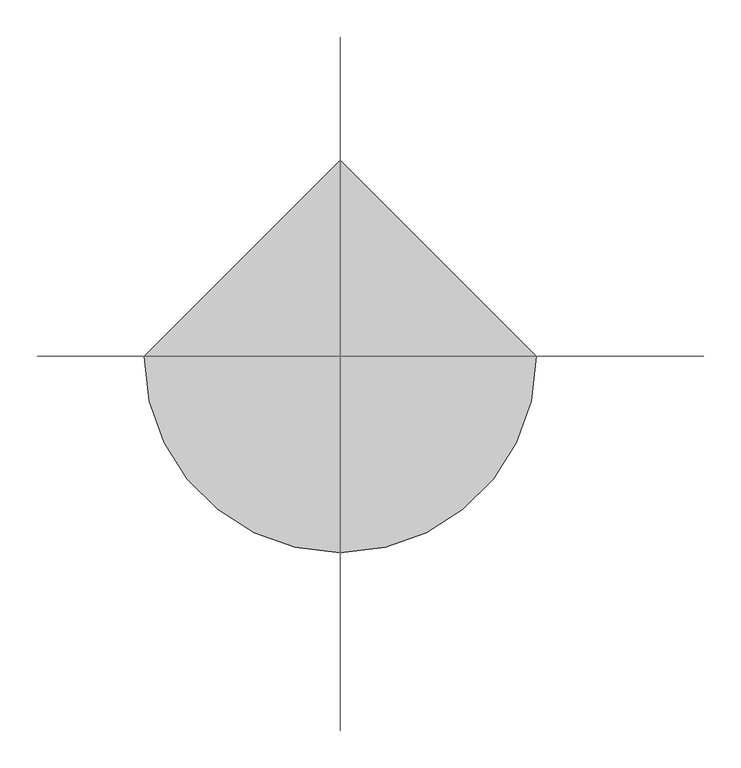
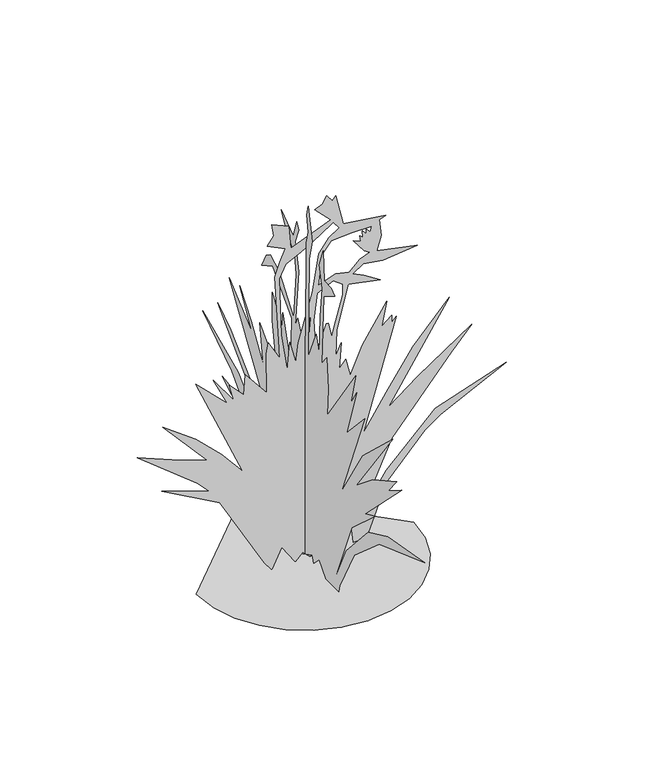
"""IFC4 building model written with IfcOpenShell, lengths in millimetres: proxy geometry, crane lily 26101 : crane lily 26101."""

from ifc_helpers import new_model, si_unit, origin, place, context, project, spatial, triangles, source, transform, mapped, element, save


def entourage_55f6ff97(model_context):
    return source(origin(), model_context, "Body", "Tessellation", [
        triangles([(-264.3380075, 0.0, 0.0272524), (-257.3504617, -60.5688865, 0.0272524), (-237.4475159, -116.1916269, 0.0272524), (-206.2245489, -165.274632, 0.0272524), (-165.274632, -206.2245489, 0.0272524), (-116.1916269, -237.4475159, 0.0272524), (-60.5688865, -257.3504617, 0.0272524), (1.16e-05, -264.3380075, 0.0272524), (60.5688865, -257.3504617, 0.0272524), (116.1916269, -237.4475159, 0.0272524), (165.274632, -206.2245489, 0.0272524), (206.2245489, -165.274632, 0.0272524), (237.4475159, -116.1916269, 0.0272524), (257.3504617, -60.5688865, 0.0272524), (264.3380075, 2.31e-05, 0.0272524), (-3.47e-05, 264.3380075, 0.0272524), (-5.2e-06, -141.3706678, 0.0), (-2.8e-06, -89.4159448, 0.054498), (-3.14e-05, -59.9343958, 33.2735186), (-3.1e-05, -36.3827356, 9.846953), (-3.03e-05, -30.3380374, 26.1345898), (2.2e-06, 22.1351019, 0.0353721), (-2.75e-05, 35.0893666, 22.475361), (-2.7e-05, 50.4325003, 13.9824575), (-2.41e-05, 71.8028075, 80.7852761), (5.2e-06, 91.613049, 0.0211753), (-2.36e-05, 109.0153662, 40.8424698), (-2.42e-05, 112.8357816, 15.9965016), (-1.83e-05, 164.4437961, 134.5614359), (-1.5e-05, 201.3025201, 190.8125718), (-8.6e-06, 314.8967674, 236.0083596), (-6.4e-06, 348.2342674, 257.8737037), (-8.8e-06, 301.5160253, 250.5209003), (-1.18e-05, 246.732487, 231.9590791), (-7.1e-06, 309.0598417, 295.0364789), (8e-07, 430.3017509, 376.6543714), (-7.9e-06, 280.4721063, 309.3519387), (-1.58e-05, 174.5674878, 204.3200503), (-9.8e-06, 240.1660818, 307.4037292), (-3e-07, 367.670363, 434.9626582), (-3.8e-06, 312.5929836, 399.2629114), (-1.14e-05, 210.1351387, 300.3374635), (-1.65e-05, 148.1844779, 220.8381918), (-1.17e-05, 187.1702069, 323.3016323), (3e-07, 320.1596366, 527.8276657), (-6.4e-06, 222.976615, 445.7627257), (-1.5e-06, 274.807899, 534.3072121), (-5.5e-06, 226.7299833, 472.9153562), (-1.02e-05, 175.4651256, 391.7724529), (-6.5e-06, 190.5821898, 491.1144633), (-1.2e-05, 119.3145649, 415.5265626), (-7.8e-06, 137.4532288, 529.6031387), (-5.6e-06, 138.7511692, 601.2540341), (-9.5e-06, 94.9513718, 536.1969586), (-8.4e-06, 93.3989229, 575.3383922), (-1.32e-05, 59.5732078, 463.4487828), (-9.8e-06, 56.2066891, 583.9388483), (-3.7e-06, 136.0049161, 669.1432405), (-2.4e-06, 181.9436545, 644.4467829), (-2.1e-06, 163.9243692, 680.6875214), (-2.5e-06, 147.0399529, 691.5511024), (-4.8e-06, 108.1804607, 671.9067347), (-1e-05, 48.046931, 590.4565101), (-6.9e-06, 36.8709235, 709.0745968), (-5.3e-06, 43.8627887, 753.7100264), (-2e-06, 83.7514831, 804.4440662), (-3e-07, 99.8779606, 836.6538008), (-3.7e-06, 49.136086, 799.8898384), (-2.9e-06, 35.0893666, 845.2923723), (-3.8e-06, 26.4505657, 828.0152292), (-4.3e-06, 41.5678933, 791.3020632), (-7e-06, 26.8495989, 721.233593), (-1.07e-05, 41.5678933, 575.3383922), (-1.05e-05, 30.7698379, 599.0950453), (-1.29e-05, 9.1735731, 551.5843188), (-1.27e-05, -4.2437592, 577.167205), (-5.7e-06, -6.2811965, 815.731822), (-5.1e-06, -13.569935, 847.4513248), (-3.6e-06, -6.9461944, 887.7586756), (-3.1e-06, -14.582304, 914.4007267), (-6.2e-06, -30.3001922, 833.2324253), (-7.2e-06, -17.1413308, 780.7407166), (-1.46e-05, -14.582304, 527.8276657), (-1.38e-05, -46.9765748, 605.5745916), (-1.57e-05, -59.9343958, 560.222854), (-1.28e-05, -63.7807226, 662.0591526), (-1.1e-05, -73.6229771, 738.5157503), (-8.8e-06, -59.9343958, 791.3020632), (-8.5e-06, -68.5729447, 815.05868), (-8.2e-06, -77.2114935, 838.812826), (-1.06e-05, -81.5307611, 763.227396), (-1.2e-05, -110.9300204, 761.8202871), (-1.3e-05, -126.4778813, 751.5510738), (-1.23e-05, -100.3333834, 735.2899298), (-1.17e-05, -79.708316, 722.0590513), (-1.66e-05, -70.7324513, 545.1047725), (-1.68e-05, -92.3897821, 572.3361045), (-1.94e-05, -98.8076044, 495.4324774), (-2.12e-05, -94.4883277, 426.3240867), (-2.14e-05, -213.2677237, 599.0950453), (-2.3e-05, -193.8311193, 517.0301053), (-2.28e-05, -217.5869913, 558.0613217), (-2.48e-05, -176.5542669, 430.6446442), (-2.57e-05, -252.1411685, 512.7095841), (-2.87e-05, -152.798395, 264.3532501), (-2.83e-05, -244.4081376, 413.0424482), (-3.04e-05, -369.3264393, 531.0712541), (-2.98e-05, -215.4274755, 318.343541), (-3.13e-05, -285.475907, 376.1107999), (-3.42e-05, -387.58906, 431.8587779), (-3.39e-05, -351.4829427, 387.4518954), (-3.53e-05, -406.9616784, 422.1127885), (-3.3e-05, -254.1018046, 269.3443517), (-3.43e-05, -295.3336628, 288.109885), (-3.26e-05, -197.6014924, 198.8161167), (-3.48e-05, -118.2442087, 7.3579794), (-3.37e-05, -173.2017281, 125.4509545), (-3.48e-05, -266.8272088, 229.6761334), (-3.73e-05, -347.9879162, 267.302198), (-4.35e-05, -504.8177693, 294.5894314), (-3.69e-05, -312.1281501, 226.3418711), (-3.5e-05, -207.3218293, 133.5593986), (-3.57e-05, -146.3193573, 18.1561127), (117.3305654, 2.31e-05, 0.0405123), (110.3389591, 2.08e-05, 74.4091073), (78.0842327, 2.54e-05, 21.0145808), (55.6151237, 2.49e-05, 46.2313396), (12.5873108, 2.89e-05, 0.0122306), (-5.1707583, 2.92e-05, 18.1490262), (-24.1045425, 3.09e-05, 0.0037426), (-56.6857342, 2.97e-05, 48.3908508), (-81.2114855, 3.28e-05, 0.0181663), (-98.986418, 3.3e-05, 24.1438615), (-207.7917316, 2.63e-05, 216.6390658), (-348.2342674, 2.78e-05, 294.5894314), (-233.774666, 2.51e-05, 255.7146967), (-261.6024369, 2.45e-05, 285.2828592), (-408.7041229, 2.4e-05, 402.5700133), (-324.6782925, 2.24e-05, 368.0386909), (-238.0939517, 2.05e-05, 335.6206115), (-346.0752786, 1.79e-05, 458.719275), (-266.2303157, 1.79e-05, 400.2179767), (-203.8244956, 1.88e-05, 339.715129), (-151.7089902, 2.02e-05, 277.3123428), (-266.1693456, 9.5e-06, 540.784215), (-189.3886398, 1.06e-05, 466.0141786), (-222.976615, 7.9e-06, 536.4662009), (-173.7341084, 9.8e-06, 467.1774796), (-184.1031521, 7.7e-06, 510.5505589), (-149.5492202, 8.4e-06, 473.8373929), (-145.2299525, 5.2e-06, 523.5096517), (-93.3989229, 6.8e-06, 458.719275), (-94.0984351, 9e-07, 559.4354384), (-89.0799006, -9e-07, 586.138496), (-61.0044976, 8e-07, 536.4662009), (-64.4230889, -1.9e-06, 583.7153154), (-73.364658, -1.14e-05, 749.2980864), (-61.7167134, -1.39e-05, 783.3111992), (-47.9079951, -1.63e-05, 813.4864649), (-91.2394163, -1.57e-05, 834.4947756), (-76.5455003, -1.76e-05, 856.3946743), (-80.4413563, -1.92e-05, 886.3260595), (-39.8899707, -2e-05, 869.0464457), (-35.0893666, -1.67e-05, 810.7381588), (62.093907, -2.33e-05, 849.6128935), (23.2207756, -2.39e-05, 888.4850847), (42.4165107, -2.52e-05, 896.5013105), (53.4556125, -2.67e-05, 914.4007267), (66.1944834, -2.63e-05, 896.8848627), (74.7598808, -2.72e-05, 906.7806976), (93.6785752, -2.34e-05, 828.1498867), (196.1872255, -2.7e-05, 813.9157265), (180.8732984, -2.6e-05, 808.5791336), (185.7325766, -2.37e-05, 766.8723043), (174.394515, -2.11e-05, 730.8322803), (273.7385602, -2.41e-05, 709.2371595), (189.3833167, -2e-05, 700.9592491), (142.0676456, -1.83e-05, 708.1576469), (116.0844387, -1.62e-05, 691.9600891), (142.8525086, -1.66e-05, 679.102589), (183.0330503, -1.68e-05, 653.0853544), (105.3178811, -1.44e-05, 669.0848139), (77.0491851, -6.7e-06, 560.5047772), (75.051728, -2.7e-06, 495.4324774), (87.9216592, -5e-06, 524.393573), (83.6900225, -9e-07, 458.719275), (98.8076044, -2.7e-06, 478.1553706), (109.6056554, -5e-07, 432.803633), (138.9439536, -5.8e-06, 499.7708027), (199.0078928, -1.39e-05, 592.0084502), (187.352336, -9.8e-06, 532.1482232), (211.1082079, -1.2e-05, 551.5843188), (211.1082079, -1.1e-05, 534.3072121), (221.9062589, -1.21e-05, 545.1047725), (142.0000807, 7.6e-06, 272.9918035), (197.3987977, 1e-07, 358.912431), (262.4025334, -8.4e-06, 452.8214155), (351.4829427, -1.8e-05, 549.4227502), (202.4694002, 2.3e-06, 318.343541), (273.8909673, -4.1e-06, 372.7275035), (405.4757589, -1.51e-05, 460.8783002), (355.6612487, -9.6e-06, 405.7856601), (211.5270596, 6.8e-06, 235.3906284), (131.6828507, 2.08e-05, 59.5396797), (197.4798247, 1.2e-05, 158.3333043), (317.0659301, -2e-07, 275.0161712), (489.6996878, -1.12e-05, 333.4616226), (330.1571005, 5e-07, 255.2422691), (291.8284444, 3.8e-06, 227.7759587), (199.2240496, 1.38e-05, 127.0808696), (148.478864, 2.13e-05, 0.0507429), (114.3788288, -2.24e-05, 797.4488537), (63.6714996, -2.01e-05, 794.7361559), (42.3199913, -1.75e-05, 767.5631779), (31.8592449, -1.25e-05, 691.9600891), (74.6966352, -1.53e-05, 706.3237473), (107.4461487, -1.62e-05, 698.437092), (132.807564, -1.88e-05, 722.7067589), (157.1176626, -2.05e-05, 732.9912329), (143.9299774, -2.04e-05, 741.276701), (117.5705943, -2.13e-05, 776.2906248), (135.9680906, -2.16e-05, 768.3049204), (133.7021497, -2.24e-05, 783.2401279), (140.693002, -2.24e-05, 777.0983517), (139.840574, -2.33e-05, 793.4610884), (148.478864, -2.3e-05, 782.6634916), (148.8047525, -2.38e-05, 795.162874), (158.4753014, -2.36e-05, 785.4854851), (162.2614257, -2.45e-05, 797.6698431), (36.4967821, -2.03e-05, 819.0008085), (-10.5179706, -1.66e-05, 790.7762959), (-46.6034508, -1.4e-05, 773.6338102), (-62.8378705, -1.14e-05, 741.9143074), (-57.6440741, -2.8e-06, 594.8100597), (-43.7276589, 2.2e-06, 499.7530349), (-37.2488755, -2.2e-06, 568.8613893), (-22.1313685, 5e-07, 512.7095841), (-15.8925131, -2.6e-06, 559.8647), (18.0916476, -1.1e-05, 677.0451565), (33.6138798, -1.74e-05, 772.2038103), (57.6697312, -2.04e-05, 805.3914648), (83.6900225, -2.25e-05, 821.5356829), (68.5729447, -2.3e-05, 840.9743219), (30.2087529, -1.13e-05, 671.65784), (21.8014718, -6.9e-06, 605.0462809), (25.6817059, -2.5e-06, 528.0867342), (30.8554363, -2.8e-06, 528.7344418), (51.5501011, -7.1e-06, 586.290885), (56.0771503, -7.3e-06, 585.6457209), (65.1309854, -5.4e-06, 548.1349654), (69.6580301, -6.8e-06, 568.1831966), (91.6460685, -1.24e-05, 645.7879074), (91.6460685, -1.4e-05, 672.9507116), (68.3644091, -1.4e-05, 690.4106197), (6.9271952, -5.7e-06, 595.3460009), (10.8074288, -4.5e-06, 573.3571904), (13.394269, -6.1e-06, 597.9317079), (15.3343985, -7.9e-06, 627.035055)], [[15, 16, 1], [14, 15, 1], [14, 1, 2], [13, 14, 2], [13, 2, 3], [13, 3, 4], [12, 13, 4], [11, 12, 4], [11, 4, 5], [11, 5, 6], [11, 6, 7], [11, 7, 8], [11, 8, 9], [11, 9, 10], [46, 47, 48], [119, 120, 121], [35, 36, 37], [106, 107, 108], [39, 40, 41], [39, 41, 42], [101, 102, 103], [111, 112, 113], [105, 106, 108], [44, 45, 46], [113, 114, 115], [54, 55, 56], [103, 104, 105], [99, 100, 101], [109, 110, 111], [89, 90, 91], [118, 119, 121], [31, 32, 33], [46, 48, 49], [44, 46, 49], [79, 80, 81], [78, 79, 81], [66, 67, 68], [27, 28, 29], [52, 53, 54], [88, 89, 91], [87, 88, 91], [49, 50, 51], [58, 59, 60], [99, 101, 103], [25, 26, 27], [83, 84, 85], [109, 111, 113], [108, 109, 113], [96, 97, 98], [68, 69, 70], [68, 70, 71], [38, 39, 42], [38, 42, 43], [65, 66, 68], [65, 68, 71], [65, 71, 72], [64, 65, 72], [64, 72, 73], [63, 64, 73], [118, 121, 122], [117, 118, 122], [117, 122, 123], [116, 117, 123], [73, 74, 75], [116, 123, 17], [116, 17, 18], [58, 60, 61], [58, 61, 62], [57, 58, 62], [57, 62, 63], [77, 78, 81], [77, 81, 82], [76, 77, 82], [76, 82, 83], [75, 76, 83], [92, 93, 94], [19, 20, 21], [30, 31, 33], [30, 33, 34], [91, 92, 94], [87, 91, 94], [87, 94, 95], [86, 87, 95], [86, 95, 96], [85, 86, 96], [34, 35, 37], [34, 37, 38], [30, 34, 38], [25, 27, 29], [57, 63, 73], [56, 57, 73], [56, 73, 75], [56, 75, 83], [23, 24, 25], [99, 103, 105], [29, 30, 38], [105, 108, 113], [105, 113, 115], [51, 52, 54], [51, 54, 56], [83, 85, 96], [21, 22, 23], [83, 96, 98], [83, 98, 99], [56, 83, 99], [29, 38, 43], [25, 29, 43], [115, 116, 18], [115, 18, 19], [105, 115, 19], [21, 23, 25], [44, 49, 51], [43, 44, 51], [56, 99, 105], [51, 56, 105], [43, 51, 105], [43, 105, 19], [25, 43, 19], [21, 25, 19], [248, 124, 125], [241, 229, 212], [206, 207, 208], [197, 198, 199], [146, 147, 148], [134, 135, 136], [196, 197, 199], [241, 212, 213], [255, 237, 238], [140, 141, 142], [200, 201, 202], [137, 138, 139], [255, 238, 239], [258, 255, 239], [175, 176, 177], [184, 185, 186], [235, 236, 237], [180, 181, 182], [189, 190, 191], [144, 145, 146], [140, 142, 143], [247, 248, 125], [171, 172, 173], [200, 202, 203], [199, 200, 203], [193, 194, 195], [237, 255, 256], [220, 221, 222], [148, 149, 150], [137, 139, 140], [224, 225, 226], [229, 241, 242], [195, 196, 199], [222, 223, 224], [153, 154, 155], [179, 180, 182], [150, 151, 152], [226, 227, 228], [191, 192, 193], [186, 187, 188], [169, 170, 171], [175, 177, 178], [152, 153, 155], [195, 199, 203], [161, 162, 163], [240, 241, 213], [240, 213, 214], [165, 166, 167], [167, 168, 169], [165, 167, 169], [165, 169, 171], [191, 193, 195], [189, 191, 195], [188, 189, 195], [239, 240, 214], [239, 214, 215], [125, 126, 127], [124, 248, 249], [124, 249, 250], [161, 163, 164], [160, 161, 164], [159, 160, 164], [131, 132, 133], [144, 146, 148], [129, 130, 131], [131, 133, 134], [206, 208, 209], [205, 206, 209], [205, 209, 210], [204, 205, 210], [204, 210, 211], [204, 211, 124], [204, 124, 250], [246, 247, 125], [195, 203, 204], [144, 148, 150], [144, 150, 152], [158, 159, 164], [127, 128, 129], [246, 125, 127], [246, 127, 129], [246, 129, 131], [136, 137, 140], [136, 140, 143], [136, 143, 144], [134, 136, 144], [131, 134, 144], [220, 222, 224], [220, 224, 226], [220, 226, 228], [219, 220, 228], [131, 144, 152], [258, 239, 215], [174, 175, 178], [186, 188, 195], [215, 216, 217], [131, 152, 155], [157, 158, 164], [217, 218, 219], [186, 195, 204], [219, 228, 229], [245, 246, 131], [245, 131, 215], [244, 245, 215], [254, 244, 215], [254, 215, 217], [253, 254, 217], [252, 253, 217], [257, 258, 215], [184, 186, 204], [184, 204, 250], [183, 184, 250], [183, 250, 251], [182, 183, 251], [182, 251, 252], [182, 252, 217], [179, 182, 217], [179, 217, 219], [178, 179, 219], [174, 178, 219], [174, 219, 229], [173, 174, 229], [171, 173, 229], [171, 229, 242], [165, 171, 242], [165, 242, 243], [165, 243, 230], [164, 165, 230], [164, 230, 231], [164, 231, 232], [157, 164, 232], [157, 232, 233], [156, 157, 233], [156, 233, 234], [156, 234, 235], [155, 156, 235], [131, 155, 235], [131, 235, 237], [131, 237, 256], [215, 131, 256], [257, 215, 256]], closed=False),
    ])


if __name__ == "__main__":
    model = new_model("IFC4")
    model_context = context("Model", 3, world=origin())
    ifc_project = project(units=[si_unit("LENGTHUNIT", "METRE", prefix="MILLI")], contexts=[model_context])
    site = spatial("IfcSite", under=ifc_project)
    building = spatial("IfcBuilding", under=site)
    placement = place(None, origin())
    entourage_shape = entourage_55f6ff97(model_context)
    element("IfcBuildingElementProxy", 1, Name="crane lily 26101 : crane lily 26101", ObjectType="crane lily 26101 : crane lily 26101", at=placement, inside=building, context=model_context, shape_type="MappedRepresentation", body=[
        mapped(entourage_shape, transform((0.0, 0.0, 0.0), x_axis=(1.0, 0.0, 0.0), y_axis=(0.0, 1.0, 0.0), z_axis=(0.0, 0.0, 1.0))),
    ])
    save(model, "model.ifc")

# Revit data of these elements
# Type "crane lily 26101 : crane lily 26101"
#   built-in parameter 1005195 = "RPC-16-FWM5-GM7X-C67P-4000-ST1L-LVER-AU"
#   Height = 0
